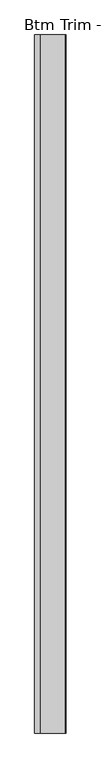
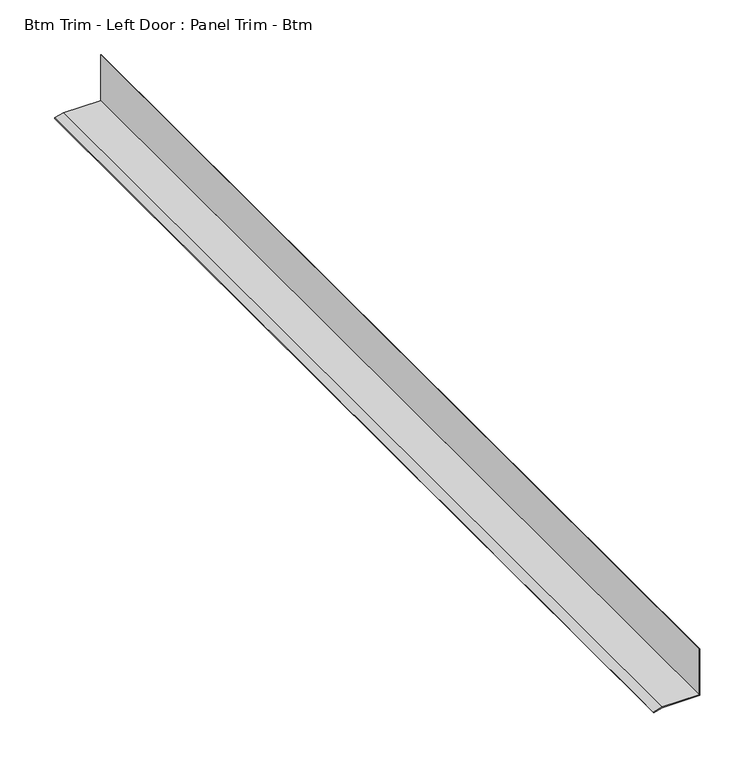
"""IFC4 building model written with IfcOpenShell, lengths in millimetres: proxy geometry, Btm Trim - Left Door : Panel Trim - Btm."""

from ifc_helpers import new_model, si_unit, frame, origin, place, context, project, spatial, polyline, outline, extrude, source, transform, mapped, element, save


def btm_trim_left_door_panel_trim_btm_813b1cb6(model_context):
    return source(origin(), model_context, "Body", "SweptSolid", [
        extrude(outline(polyline([(50.8, 587326.1141748), (48.3077022, 587316.8127928), (47.5409986, 587317.0182304), (50.00625, 587326.2186739), (50.00625, 587365.8934739), (101.6, 587365.8934739), (101.6, 587365.1060739), (50.8, 587365.1060739), (50.8, 587326.1141748)])), frame((0.0, -532878.2537841, 0.0), z_axis=(0.0, 1.0, 0.0), x_axis=(0.0, 0.0, 1.0)), (0.0, 0.0, 1.0), 1093.7880247),
    ])


if __name__ == "__main__":
    model = new_model("IFC4")
    model_context = context("Model", 3, world=origin())
    ifc_project = project(units=[si_unit("LENGTHUNIT", "METRE", prefix="MILLI")], contexts=[model_context])
    site = spatial("IfcSite", under=ifc_project)
    building = spatial("IfcBuilding", under=site)
    placement = place(None, origin())
    btm_trim_left_door_panel_trim_btm_shape = btm_trim_left_door_panel_trim_btm_813b1cb6(model_context)
    element("IfcBuildingElementProxy", 1, Name="Btm Trim - Left Door : Panel Trim - Btm", ObjectType="Btm Trim - Left Door : Panel Trim - Btm", at=placement, inside=building, context=model_context, shape_type="MappedRepresentation", body=[
        mapped(btm_trim_left_door_panel_trim_btm_shape, transform((0.0, 0.0, 0.0), x_axis=(1.0, 0.0, 0.0), y_axis=(0.0, 1.0, 0.0), z_axis=(0.0, 0.0, 1.0))),
    ])
    save(model, "model.ifc")

# Revit data of these elements
# Element 1 (IfcBuildingElementProxy, "Btm Trim - Left Door : Panel Trim - Btm")
#   Materials on its faces: "BASE TRIM BY MTL PANEL MFR."
# Materials
#   "BASE TRIM BY MTL PANEL MFR.": class "Generic", colour RGB 239 242 240, transparency 0, Cost = 0
